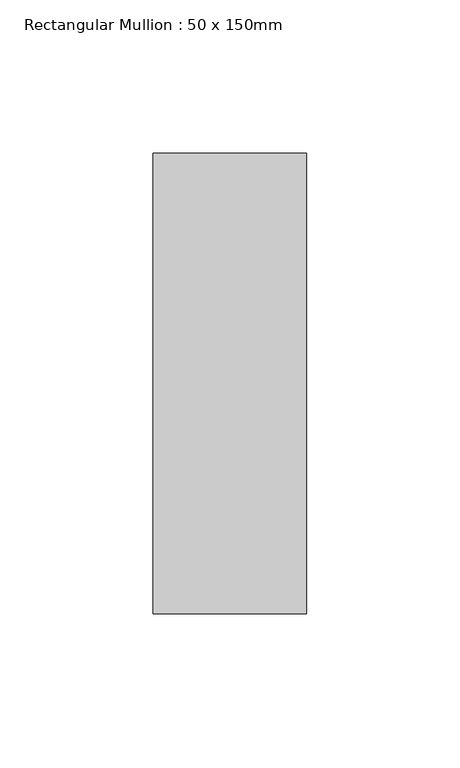
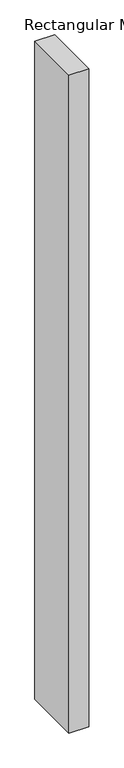
"""IFC4 building model written with IfcOpenShell, lengths in millimetres: member geometry, Rectangular Mullion : 50 x 150mm."""

from ifc_helpers import new_model, si_unit, frame, origin, place, context, project, spatial, polyline, outline, extrude, source, transform, mapped, element, save


def rectangular_mullion_50_x_150mm_14f53fa3(model_context):
    return source(origin(), model_context, "Body", "SweptSolid", [
        extrude(outline(polyline([(25.0, 75.0), (25.0, -75.0), (-25.0, -75.0), (-25.0, 75.0), (25.0, 75.0)])), frame((0.0, 0.0, -1767.0), z_axis=(0.0, 0.0, 1.0), x_axis=(1.0, 0.0, 0.0)), (0.0, 0.0, 1.0), 1767.0),
    ])


if __name__ == "__main__":
    model = new_model("IFC4")
    model_context = context("Model", 3, world=origin())
    ifc_project = project(units=[si_unit("LENGTHUNIT", "METRE", prefix="MILLI")], contexts=[model_context])
    site = spatial("IfcSite", under=ifc_project)
    building = spatial("IfcBuilding", under=site)
    placement = place(None, origin())
    rectangular_mullion_50_x_150mm_shape = rectangular_mullion_50_x_150mm_14f53fa3(model_context)
    element("IfcMember", 1, ObjectType="Rectangular Mullion : 50 x 150mm", at=placement, inside=building, context=model_context, shape_type="MappedRepresentation", body=[
        mapped(rectangular_mullion_50_x_150mm_shape, transform((0.0, 0.0, 0.0), x_axis=(1.0, 0.0, 0.0), y_axis=(0.0, 1.0, 0.0), z_axis=(0.0, 0.0, 1.0))),
    ])
    save(model, "model.ifc")

# Revit data of these elements
# Type "Rectangular Mullion : 50 x 150mm"
#   Keynote = "H11"
#   built-in parameter 1007304 = 0.492126 (stored number, unit not read)
#   built-in parameter 1007301 = 0.082021 (stored number, unit not read)
#   built-in parameter 1007300 = 0.082021 (stored number, unit not read)
# Element 1 (IfcMember, "Rectangular Mullion : 50 x 150mm")
#   Materials on its faces: "Aluminium"
# Materials
#   "Aluminium": class "Metal", colour RGB 247 247 247, transparency 0, Description = "Aluminium 6061", Cost = 0
